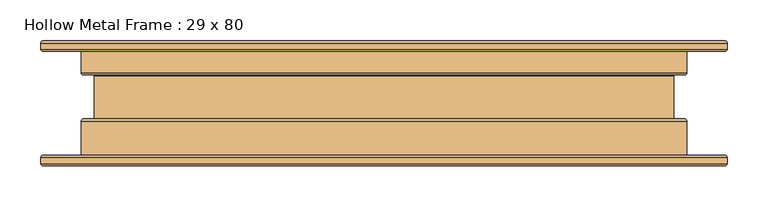
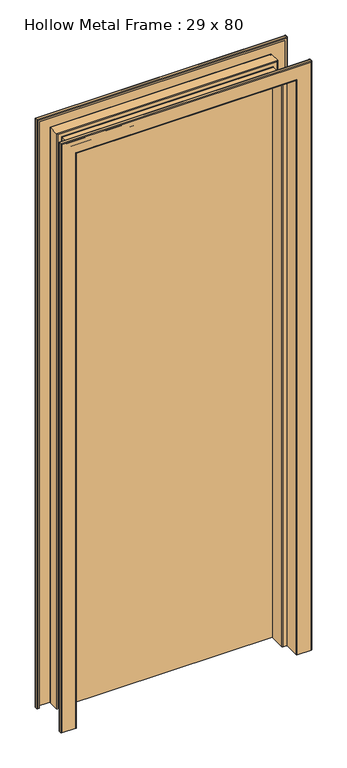
"""IFC4 building model written with IfcOpenShell, lengths in millimetres: door geometry, Hollow Metal Frame : 29 x 80."""

from ifc_helpers import new_model, si_unit, frame, origin, origin_with_axes, place, context, project, spatial, polyline, circle_curve, ellipse_curve, outline, extrude, source, transform, mapped, element, save
from ifc_brep_helpers import plane_surface, cylinder_surface, revolved_surface, advanced_brep


def hollow_metal_frame_29_x_80_a7873af5(model_context):
    return source(origin(), model_context, "Body", "SolidModel", [
        advanced_brep(
        [(-416.52825, -63.5635, 0.0), (-411.1625, -63.5635, 0.0), (-411.1625, -65.11925, 0.0), (-416.52825, -65.11925, 0.0), (-417.54425, -66.13525, 0.0), (-417.54425, -73.66, 0.0), (-416.52825, -74.676, 0.0), (-370.87175, -74.676, 0.0), (-369.85575, -73.66, 0.0), (-369.85575, -21.68525, 0.0), (-367.284, -19.1135, 0.0), (-354.99675, -19.1135, 0.0), (-353.98075, -18.0975, 0.0), (-353.98075, 33.6931, 0.0), (-354.99675, 34.7091, 0.0), (-367.284, 34.7091, 0.0), (-369.85575, 37.28085, 0.0), (-369.85575, 73.5965, 0.0), (-370.87175, 74.6125, 0.0), (-416.52825, 74.6125, 0.0), (-417.54425, 73.5965, 0.0), (-417.54425, 66.07175, 0.0), (-416.52825, 65.05575, 0.0), (-411.1625, 65.05575, 0.0), (-411.1625, 63.5, 0.0), (-416.52825, 63.5, 0.0), (-419.1, 66.07175, 0.0), (-419.1, 73.5965, 0.0), (-416.52825, 76.16825, 0.0), (-370.87175, 76.16825, 0.0), (-368.3, 73.5965, 0.0), (-368.3, 37.28085, 0.0), (-367.284, 36.26485, 0.0), (-354.99675, 36.26485, 0.0), (-352.425, 33.6931, 0.0), (-352.425, -18.0975, 0.0), (-354.99675, -20.66925, 0.0), (-367.284, -20.66925, 0.0), (-368.3, -21.68525, 0.0), (-368.3, -73.66, 0.0), (-370.87175, -76.23175, 0.0), (-416.52825, -76.23175, 0.0), (-419.1, -73.66, 0.0), (-419.1, -66.13525, 0.0), (-419.1, -66.13525, 2082.8000001), (-416.52825, -63.5635, 2080.2282501), (-419.1, -73.66, 2082.8000001), (-416.52825, -76.23175, 2080.2282501), (-370.87175, -76.23175, 2034.5717501), (370.87175, -76.23175, 2034.5717501), (370.87175, -76.23175, 0.0), (416.52825, -76.23175, 0.0), (416.52825, -76.23175, 2080.2282501), (-368.3, -73.66, 2032.0000001), (-368.3, -21.68525, 2032.0000001), (-367.284, -20.66925, 2030.9840001), (-354.99675, -20.66925, 2018.6967501), (354.99675, -20.66925, 2018.6967501), (354.99675, -20.66925, 0.0), (367.284, -20.66925, 0.0), (367.284, -20.66925, 2030.9840001), (-352.425, -18.0975, 2016.1250001), (-352.425, 33.6931, 2016.1250001), (-354.99675, 36.26485, 2018.6967501), (-367.284, 36.26485, 2030.9840001), (367.284, 36.26485, 2030.9840001), (367.284, 36.26485, 0.0), (354.99675, 36.26485, 0.0), (354.99675, 36.26485, 2018.6967501), (-368.3, 37.28085, 2032.0000001), (-368.3, 73.5965, 2032.0000001), (-370.87175, 76.16825, 2034.5717501), (-416.52825, 76.16825, 2080.2282501), (416.52825, 76.16825, 2080.2282501), (416.52825, 76.16825, 0.0), (370.87175, 76.16825, 0.0), (370.87175, 76.16825, 2034.5717501), (-419.1, 73.5965, 2082.8000001), (-419.1, 66.07175, 2082.8000001), (-416.52825, 63.5, 2080.2282501), (-411.1625, 63.5, 2074.8625001), (411.1625, 63.5, 2074.8625001), (411.1625, 63.5, 0.0), (416.52825, 63.5, 0.0), (416.52825, 63.5, 2080.2282501), (-411.1625, 65.05575, 2074.8625001), (-416.52825, 65.05575, 2080.2282501), (416.52825, 65.05575, 2080.2282501), (416.52825, 65.05575, 0.0), (411.1625, 65.05575, 0.0), (411.1625, 65.05575, 2074.8625001), (-417.54425, 66.07175, 2081.2442501), (-417.54425, 73.5965, 2081.2442501), (-416.52825, 74.6125, 2080.2282501), (-370.87175, 74.6125, 2034.5717501), (370.87175, 74.6125, 2034.5717501), (370.87175, 74.6125, 0.0), (416.52825, 74.6125, 0.0), (416.52825, 74.6125, 2080.2282501), (-369.85575, 73.5965, 2033.5557501), (-369.85575, 37.28085, 2033.5557501), (-367.284, 34.7091, 2030.9840001), (-354.99675, 34.7091, 2018.6967501), (354.99675, 34.7091, 2018.6967501), (354.99675, 34.7091, 0.0), (367.284, 34.7091, 0.0), (367.284, 34.7091, 2030.9840001), (-353.98075, 33.6931, 2017.6807501), (-353.98075, -18.0975, 2017.6807501), (-354.99675, -19.1135, 2018.6967501), (-367.284, -19.1135, 2030.9840001), (367.284, -19.1135, 2030.9840001), (367.284, -19.1135, 0.0), (354.99675, -19.1135, 0.0), (354.99675, -19.1135, 2018.6967501), (-369.85575, -21.68525, 2033.5557501), (-369.85575, -73.66, 2033.5557501), (-370.87175, -74.676, 2034.5717501), (-416.52825, -74.676, 2080.2282501), (416.52825, -74.676, 2080.2282501), (416.52825, -74.676, 0.0), (370.87175, -74.676, 0.0), (370.87175, -74.676, 2034.5717501), (-417.54425, -73.66, 2081.2442501), (-417.54425, -66.13525, 2081.2442501), (-416.52825, -65.11925, 2080.2282501), (-411.1625, -65.11925, 2074.8625001), (411.1625, -65.11925, 2074.8625001), (411.1625, -65.11925, 0.0), (416.52825, -65.11925, 0.0), (416.52825, -65.11925, 2080.2282501), (-411.1625, -63.5635, 2074.8625001), (416.52825, -63.5635, 2080.2282501), (416.52825, -63.5635, 0.0), (411.1625, -63.5635, 0.0), (411.1625, -63.5635, 2074.8625001), (419.1, -66.13525, 2082.8000001), (419.1, -73.66, 2082.8000001), (368.3, -73.66, 2032.0000001), (368.3, -21.68525, 2032.0000001), (352.425, -18.0975, 2016.1250001), (352.425, 33.6931, 2016.1250001), (368.3, 37.28085, 2032.0000001), (368.3, 73.5965, 2032.0000001), (419.1, 73.5965, 2082.8000001), (419.1, 66.07175, 2082.8000001), (417.54425, 66.07175, 2081.2442501), (417.54425, 73.5965, 2081.2442501), (369.85575, 73.5965, 2033.5557501), (369.85575, 37.28085, 2033.5557501), (353.98075, 33.6931, 2017.6807501), (353.98075, -18.0975, 2017.6807501), (369.85575, -21.68525, 2033.5557501), (369.85575, -73.66, 2033.5557501), (417.54425, -73.66, 2081.2442501), (417.54425, -66.13525, 2081.2442501), (419.1, -66.13525, 0.0), (419.1, -73.66, 0.0), (368.3, -73.66, 0.0), (368.3, -21.68525, 0.0), (352.425, -18.0975, 0.0), (352.425, 33.6931, 0.0), (368.3, 37.28085, 0.0), (368.3, 73.5965, 0.0), (419.1, 73.5965, 0.0), (419.1, 66.07175, 0.0), (417.54425, 66.07175, 0.0), (417.54425, 73.5965, 0.0), (369.85575, 73.5965, 0.0), (369.85575, 37.28085, 0.0), (353.98075, 33.6931, 0.0), (353.98075, -18.0975, 0.0), (369.85575, -21.68525, 0.0), (369.85575, -73.66, 0.0), (417.54425, -73.66, 0.0), (417.54425, -66.13525, 0.0)],
        [
            (0, 1),
            (1, 2),
            (2, 3),
            (3, 4, circle_curve(frame((-416.52825, -66.13525, 0.0), z_axis=(0.0, 0.0, 1.0), x_axis=(0.0, 1.0, 0.0)), 1.016)),
            (4, 5),
            (5, 6, circle_curve(frame((-416.52825, -73.66, 0.0), z_axis=(0.0, 0.0, 1.0), x_axis=(0.0, 1.0, 0.0)), 1.016)),
            (6, 7),
            (7, 8, circle_curve(frame((-370.87175, -73.66, 0.0), z_axis=(0.0, 0.0, 1.0), x_axis=(0.0, 1.0, 0.0)), 1.016)),
            (8, 9),
            (9, 10, circle_curve(frame((-367.284, -21.68525, 0.0), z_axis=(0.0, 0.0, -1.0), x_axis=(0.0, 1.0, 0.0)), 2.57175)),
            (10, 11),
            (11, 12, circle_curve(frame((-354.99675, -18.0975, 0.0), z_axis=(0.0, 0.0, 1.0), x_axis=(0.0, 1.0, 0.0)), 1.016)),
            (12, 13),
            (13, 14, circle_curve(frame((-354.99675, 33.6931, 0.0), z_axis=(0.0, 0.0, 1.0), x_axis=(0.0, 1.0, 0.0)), 1.016)),
            (14, 15),
            (15, 16, circle_curve(frame((-367.284, 37.28085, 0.0), z_axis=(0.0, 0.0, -1.0), x_axis=(0.0, 1.0, 0.0)), 2.57175)),
            (16, 17),
            (17, 18, circle_curve(frame((-370.87175, 73.5965, 0.0), z_axis=(0.0, 0.0, 1.0), x_axis=(0.0, 1.0, 0.0)), 1.016)),
            (18, 19),
            (19, 20, circle_curve(frame((-416.52825, 73.5965, 0.0), z_axis=(0.0, 0.0, 1.0), x_axis=(0.0, 1.0, 0.0)), 1.016)),
            (20, 21),
            (21, 22, circle_curve(frame((-416.52825, 66.07175, 0.0), z_axis=(0.0, 0.0, 1.0), x_axis=(0.0, 1.0, 0.0)), 1.016)),
            (22, 23),
            (23, 24),
            (24, 25),
            (25, 26, circle_curve(frame((-416.52825, 66.07175, 0.0), z_axis=(0.0, 0.0, -1.0), x_axis=(0.0, 1.0, 0.0)), 2.57175)),
            (26, 27),
            (27, 28, circle_curve(frame((-416.52825, 73.5965, 0.0), z_axis=(0.0, 0.0, -1.0), x_axis=(0.0, 1.0, 0.0)), 2.57175)),
            (28, 29),
            (29, 30, circle_curve(frame((-370.87175, 73.5965, 0.0), z_axis=(0.0, 0.0, -1.0), x_axis=(0.0, 1.0, 0.0)), 2.57175)),
            (30, 31),
            (31, 32, circle_curve(frame((-367.284, 37.28085, 0.0), z_axis=(0.0, 0.0, 1.0), x_axis=(0.0, 1.0, 0.0)), 1.016)),
            (32, 33),
            (33, 34, circle_curve(frame((-354.99675, 33.6931, 0.0), z_axis=(0.0, 0.0, -1.0), x_axis=(0.0, 1.0, 0.0)), 2.57175)),
            (34, 35),
            (35, 36, circle_curve(frame((-354.99675, -18.0975, 0.0), z_axis=(0.0, 0.0, -1.0), x_axis=(0.0, 1.0, 0.0)), 2.57175)),
            (36, 37),
            (37, 38, circle_curve(frame((-367.284, -21.68525, 0.0), z_axis=(0.0, 0.0, 1.0), x_axis=(0.0, 1.0, 0.0)), 1.016)),
            (38, 39),
            (39, 40, circle_curve(frame((-370.87175, -73.66, 0.0), z_axis=(0.0, 0.0, -1.0), x_axis=(0.0, 1.0, 0.0)), 2.57175)),
            (40, 41),
            (41, 42, circle_curve(frame((-416.52825, -73.66, 0.0), z_axis=(0.0, 0.0, -1.0), x_axis=(0.0, 1.0, 0.0)), 2.57175)),
            (42, 43),
            (43, 0, circle_curve(frame((-416.52825, -66.13525, 0.0), z_axis=(0.0, 0.0, -1.0), x_axis=(0.0, 1.0, 0.0)), 2.57175)),
            (43, 44),
            (44, 45, ellipse_curve(frame((-416.52825, -66.13525, 2080.2282501), z_axis=(-0.7071067811865475, 0.0, -0.7071067811865475), x_axis=(0.7071067811865474, 0.0, -0.7071067811865476)), 3.6370037, 2.57175)),
            (45, 0),
            (42, 46),
            (46, 44),
            (41, 47),
            (47, 46, ellipse_curve(frame((-416.52825, -73.66, 2080.2282501), z_axis=(-0.7071067811865475, 0.0, -0.7071067811865475), x_axis=(0.7071067811865474, 0.0, -0.7071067811865476)), 3.6370037, 2.57175)),
            (40, 48),
            (48, 49),
            (49, 50),
            (50, 51),
            (51, 52),
            (52, 47),
            (39, 53),
            (53, 48, ellipse_curve(frame((-370.87175, -73.66, 2034.5717501), z_axis=(-0.7071067811865475, 0.0, -0.7071067811865475), x_axis=(0.7071067811865474, 0.0, -0.7071067811865476)), 3.6370037, 2.57175)),
            (38, 54),
            (54, 53),
            (37, 55),
            (55, 54, ellipse_curve(frame((-367.284, -21.68525, 2030.9840001), z_axis=(0.7071067811865475, 0.0, 0.7071067811865475), x_axis=(-0.7071067811865474, 0.0, 0.7071067811865476)), 1.436841, 1.016)),
            (36, 56),
            (56, 57),
            (57, 58),
            (58, 59),
            (59, 60),
            (60, 55),
            (35, 61),
            (61, 56, ellipse_curve(frame((-354.99675, -18.0975, 2018.6967501), z_axis=(-0.7071067811865475, 0.0, -0.7071067811865475), x_axis=(0.7071067811865474, 0.0, -0.7071067811865476)), 3.6370037, 2.57175)),
            (34, 62),
            (62, 61),
            (33, 63),
            (63, 62, ellipse_curve(frame((-354.99675, 33.6931, 2018.6967501), z_axis=(-0.7071067811865475, 0.0, -0.7071067811865475), x_axis=(0.7071067811865474, 0.0, -0.7071067811865476)), 3.6370037, 2.57175)),
            (32, 64),
            (64, 65),
            (65, 66),
            (66, 67),
            (67, 68),
            (68, 63),
            (31, 69),
            (69, 64, ellipse_curve(frame((-367.284, 37.28085, 2030.9840001), z_axis=(0.7071067811865475, 0.0, 0.7071067811865475), x_axis=(-0.7071067811865474, 0.0, 0.7071067811865476)), 1.436841, 1.016)),
            (30, 70),
            (70, 69),
            (29, 71),
            (71, 70, ellipse_curve(frame((-370.87175, 73.5965, 2034.5717501), z_axis=(-0.7071067811865475, 0.0, -0.7071067811865475), x_axis=(0.7071067811865474, 0.0, -0.7071067811865476)), 3.6370037, 2.57175)),
            (28, 72),
            (72, 73),
            (73, 74),
            (74, 75),
            (75, 76),
            (76, 71),
            (27, 77),
            (77, 72, ellipse_curve(frame((-416.52825, 73.5965, 2080.2282501), z_axis=(-0.7071067811865475, 0.0, -0.7071067811865475), x_axis=(0.7071067811865474, 0.0, -0.7071067811865476)), 3.6370037, 2.57175)),
            (26, 78),
            (78, 77),
            (25, 79),
            (79, 78, ellipse_curve(frame((-416.52825, 66.07175, 2080.2282501), z_axis=(-0.7071067811865475, 0.0, -0.7071067811865475), x_axis=(0.7071067811865474, 0.0, -0.7071067811865476)), 3.6370037, 2.57175)),
            (24, 80),
            (80, 81),
            (81, 82),
            (82, 83),
            (83, 84),
            (84, 79),
            (23, 85),
            (85, 80),
            (22, 86),
            (86, 87),
            (87, 88),
            (88, 89),
            (89, 90),
            (90, 85),
            (21, 91),
            (91, 86, ellipse_curve(frame((-416.52825, 66.07175, 2080.2282501), z_axis=(0.7071067811865475, 0.0, 0.7071067811865475), x_axis=(-0.7071067811865474, 0.0, 0.7071067811865476)), 1.436841, 1.016)),
            (20, 92),
            (92, 91),
            (19, 93),
            (93, 92, ellipse_curve(frame((-416.52825, 73.5965, 2080.2282501), z_axis=(0.7071067811865475, 0.0, 0.7071067811865475), x_axis=(-0.7071067811865474, 0.0, 0.7071067811865476)), 1.436841, 1.016)),
            (18, 94),
            (94, 95),
            (95, 96),
            (96, 97),
            (97, 98),
            (98, 93),
            (17, 99),
            (99, 94, ellipse_curve(frame((-370.87175, 73.5965, 2034.5717501), z_axis=(0.7071067811865475, 0.0, 0.7071067811865475), x_axis=(-0.7071067811865474, 0.0, 0.7071067811865476)), 1.436841, 1.016)),
            (16, 100),
            (100, 99),
            (15, 101),
            (101, 100, ellipse_curve(frame((-367.284, 37.28085, 2030.9840001), z_axis=(-0.7071067811865475, 0.0, -0.7071067811865475), x_axis=(0.7071067811865474, 0.0, -0.7071067811865476)), 3.6370037, 2.57175)),
            (14, 102),
            (102, 103),
            (103, 104),
            (104, 105),
            (105, 106),
            (106, 101),
            (13, 107),
            (107, 102, ellipse_curve(frame((-354.99675, 33.6931, 2018.6967501), z_axis=(0.7071067811865475, 0.0, 0.7071067811865475), x_axis=(-0.7071067811865474, 0.0, 0.7071067811865476)), 1.436841, 1.016)),
            (12, 108),
            (108, 107),
            (11, 109),
            (109, 108, ellipse_curve(frame((-354.99675, -18.0975, 2018.6967501), z_axis=(0.7071067811865475, 0.0, 0.7071067811865475), x_axis=(-0.7071067811865474, 0.0, 0.7071067811865476)), 1.436841, 1.016)),
            (10, 110),
            (110, 111),
            (111, 112),
            (112, 113),
            (113, 114),
            (114, 109),
            (9, 115),
            (115, 110, ellipse_curve(frame((-367.284, -21.68525, 2030.9840001), z_axis=(-0.7071067811865475, 0.0, -0.7071067811865475), x_axis=(0.7071067811865474, 0.0, -0.7071067811865476)), 3.6370037, 2.57175)),
            (8, 116),
            (116, 115),
            (7, 117),
            (117, 116, ellipse_curve(frame((-370.87175, -73.66, 2034.5717501), z_axis=(0.7071067811865475, 0.0, 0.7071067811865475), x_axis=(-0.7071067811865474, 0.0, 0.7071067811865476)), 1.436841, 1.016)),
            (6, 118),
            (118, 119),
            (119, 120),
            (120, 121),
            (121, 122),
            (122, 117),
            (5, 123),
            (123, 118, ellipse_curve(frame((-416.52825, -73.66, 2080.2282501), z_axis=(0.7071067811865475, 0.0, 0.7071067811865475), x_axis=(-0.7071067811865474, 0.0, 0.7071067811865476)), 1.436841, 1.016)),
            (4, 124),
            (124, 123),
            (3, 125),
            (125, 124, ellipse_curve(frame((-416.52825, -66.13525, 2080.2282501), z_axis=(0.7071067811865475, 0.0, 0.7071067811865475), x_axis=(-0.7071067811865474, 0.0, 0.7071067811865476)), 1.436841, 1.016)),
            (2, 126),
            (126, 127),
            (127, 128),
            (128, 129),
            (129, 130),
            (130, 125),
            (1, 131),
            (131, 126),
            (45, 132),
            (132, 133),
            (133, 134),
            (134, 135),
            (135, 131),
            (44, 136),
            (136, 132, ellipse_curve(frame((416.52825, -66.13525, 2080.2282501), z_axis=(-0.7071067811865475, 0.0, 0.7071067811865475), x_axis=(-0.7071067811865476, 0.0, -0.7071067811865474)), 3.6370037, 2.57175)),
            (46, 137),
            (137, 136),
            (52, 137, ellipse_curve(frame((416.52825, -73.66, 2080.2282501), z_axis=(-0.7071067811865475, 0.0, 0.7071067811865475), x_axis=(-0.7071067811865476, 0.0, -0.7071067811865474)), 3.6370037, 2.57175)),
            (53, 138),
            (138, 49, ellipse_curve(frame((370.87175, -73.66, 2034.5717501), z_axis=(-0.7071067811865475, 0.0, 0.7071067811865475), x_axis=(-0.7071067811865476, 0.0, -0.7071067811865474)), 3.6370037, 2.57175)),
            (54, 139),
            (139, 138),
            (60, 139, ellipse_curve(frame((367.284, -21.68525, 2030.9840001), z_axis=(0.7071067811865475, 0.0, -0.7071067811865475), x_axis=(0.7071067811865476, 0.0, 0.7071067811865474)), 1.436841, 1.016)),
            (61, 140),
            (140, 57, ellipse_curve(frame((354.99675, -18.0975, 2018.6967501), z_axis=(-0.7071067811865475, 0.0, 0.7071067811865475), x_axis=(-0.7071067811865476, 0.0, -0.7071067811865474)), 3.6370037, 2.57175)),
            (62, 141),
            (141, 140),
            (68, 141, ellipse_curve(frame((354.99675, 33.6931, 2018.6967501), z_axis=(-0.7071067811865475, 0.0, 0.7071067811865475), x_axis=(-0.7071067811865476, 0.0, -0.7071067811865474)), 3.6370037, 2.57175)),
            (69, 142),
            (142, 65, ellipse_curve(frame((367.284, 37.28085, 2030.9840001), z_axis=(0.7071067811865475, 0.0, -0.7071067811865475), x_axis=(0.7071067811865476, 0.0, 0.7071067811865474)), 1.436841, 1.016)),
            (70, 143),
            (143, 142),
            (76, 143, ellipse_curve(frame((370.87175, 73.5965, 2034.5717501), z_axis=(-0.7071067811865475, 0.0, 0.7071067811865475), x_axis=(-0.7071067811865476, 0.0, -0.7071067811865474)), 3.6370037, 2.57175)),
            (77, 144),
            (144, 73, ellipse_curve(frame((416.52825, 73.5965, 2080.2282501), z_axis=(-0.7071067811865475, 0.0, 0.7071067811865475), x_axis=(-0.7071067811865476, 0.0, -0.7071067811865474)), 3.6370037, 2.57175)),
            (78, 145),
            (145, 144),
            (84, 145, ellipse_curve(frame((416.52825, 66.07175, 2080.2282501), z_axis=(-0.7071067811865475, 0.0, 0.7071067811865475), x_axis=(-0.7071067811865476, 0.0, -0.7071067811865474)), 3.6370037, 2.57175)),
            (90, 81),
            (91, 146),
            (146, 87, ellipse_curve(frame((416.52825, 66.07175, 2080.2282501), z_axis=(0.7071067811865475, 0.0, -0.7071067811865475), x_axis=(0.7071067811865476, 0.0, 0.7071067811865474)), 1.436841, 1.016)),
            (92, 147),
            (147, 146),
            (98, 147, ellipse_curve(frame((416.52825, 73.5965, 2080.2282501), z_axis=(0.7071067811865475, 0.0, -0.7071067811865475), x_axis=(0.7071067811865476, 0.0, 0.7071067811865474)), 1.436841, 1.016)),
            (99, 148),
            (148, 95, ellipse_curve(frame((370.87175, 73.5965, 2034.5717501), z_axis=(0.7071067811865475, 0.0, -0.7071067811865475), x_axis=(0.7071067811865476, 0.0, 0.7071067811865474)), 1.436841, 1.016)),
            (100, 149),
            (149, 148),
            (106, 149, ellipse_curve(frame((367.284, 37.28085, 2030.9840001), z_axis=(-0.7071067811865475, 0.0, 0.7071067811865475), x_axis=(-0.7071067811865476, 0.0, -0.7071067811865474)), 3.6370037, 2.57175)),
            (107, 150),
            (150, 103, ellipse_curve(frame((354.99675, 33.6931, 2018.6967501), z_axis=(0.7071067811865475, 0.0, -0.7071067811865475), x_axis=(0.7071067811865476, 0.0, 0.7071067811865474)), 1.436841, 1.016)),
            (108, 151),
            (151, 150),
            (114, 151, ellipse_curve(frame((354.99675, -18.0975, 2018.6967501), z_axis=(0.7071067811865475, 0.0, -0.7071067811865475), x_axis=(0.7071067811865476, 0.0, 0.7071067811865474)), 1.436841, 1.016)),
            (115, 152),
            (152, 111, ellipse_curve(frame((367.284, -21.68525, 2030.9840001), z_axis=(-0.7071067811865475, 0.0, 0.7071067811865475), x_axis=(-0.7071067811865476, 0.0, -0.7071067811865474)), 3.6370037, 2.57175)),
            (116, 153),
            (153, 152),
            (122, 153, ellipse_curve(frame((370.87175, -73.66, 2034.5717501), z_axis=(0.7071067811865475, 0.0, -0.7071067811865475), x_axis=(0.7071067811865476, 0.0, 0.7071067811865474)), 1.436841, 1.016)),
            (123, 154),
            (154, 119, ellipse_curve(frame((416.52825, -73.66, 2080.2282501), z_axis=(0.7071067811865475, 0.0, -0.7071067811865475), x_axis=(0.7071067811865476, 0.0, 0.7071067811865474)), 1.436841, 1.016)),
            (124, 155),
            (155, 154),
            (130, 155, ellipse_curve(frame((416.52825, -66.13525, 2080.2282501), z_axis=(0.7071067811865475, 0.0, -0.7071067811865475), x_axis=(0.7071067811865476, 0.0, 0.7071067811865474)), 1.436841, 1.016)),
            (135, 127),
            (133, 156, circle_curve(frame((416.52825, -66.13525, 0.0), z_axis=(0.0, 0.0, -1.0), x_axis=(0.0, 1.0, 0.0)), 2.57175)),
            (156, 157),
            (157, 51, circle_curve(frame((416.52825, -73.66, 0.0), z_axis=(0.0, 0.0, -1.0), x_axis=(0.0, 1.0, 0.0)), 2.57175)),
            (50, 158, circle_curve(frame((370.87175, -73.66, 0.0), z_axis=(0.0, 0.0, -1.0), x_axis=(0.0, 1.0, 0.0)), 2.57175)),
            (158, 159),
            (159, 59, circle_curve(frame((367.284, -21.68525, 0.0), z_axis=(0.0, 0.0, 1.0), x_axis=(0.0, 1.0, 0.0)), 1.016)),
            (58, 160, circle_curve(frame((354.99675, -18.0975, 0.0), z_axis=(0.0, 0.0, -1.0), x_axis=(0.0, 1.0, 0.0)), 2.57175)),
            (160, 161),
            (161, 67, circle_curve(frame((354.99675, 33.6931, 0.0), z_axis=(0.0, 0.0, -1.0), x_axis=(0.0, 1.0, 0.0)), 2.57175)),
            (66, 162, circle_curve(frame((367.284, 37.28085, 0.0), z_axis=(0.0, 0.0, 1.0), x_axis=(0.0, 1.0, 0.0)), 1.016)),
            (162, 163),
            (163, 75, circle_curve(frame((370.87175, 73.5965, 0.0), z_axis=(0.0, 0.0, -1.0), x_axis=(0.0, 1.0, 0.0)), 2.57175)),
            (74, 164, circle_curve(frame((416.52825, 73.5965, 0.0), z_axis=(0.0, 0.0, -1.0), x_axis=(0.0, 1.0, 0.0)), 2.57175)),
            (164, 165),
            (165, 83, circle_curve(frame((416.52825, 66.07175, 0.0), z_axis=(0.0, 0.0, -1.0), x_axis=(0.0, 1.0, 0.0)), 2.57175)),
            (82, 89),
            (88, 166, circle_curve(frame((416.52825, 66.07175, 0.0), z_axis=(0.0, 0.0, 1.0), x_axis=(0.0, 1.0, 0.0)), 1.016)),
            (166, 167),
            (167, 97, circle_curve(frame((416.52825, 73.5965, 0.0), z_axis=(0.0, 0.0, 1.0), x_axis=(0.0, 1.0, 0.0)), 1.016)),
            (96, 168, circle_curve(frame((370.87175, 73.5965, 0.0), z_axis=(0.0, 0.0, 1.0), x_axis=(0.0, 1.0, 0.0)), 1.016)),
            (168, 169),
            (169, 105, circle_curve(frame((367.284, 37.28085, 0.0), z_axis=(0.0, 0.0, -1.0), x_axis=(0.0, 1.0, 0.0)), 2.57175)),
            (104, 170, circle_curve(frame((354.99675, 33.6931, 0.0), z_axis=(0.0, 0.0, 1.0), x_axis=(0.0, 1.0, 0.0)), 1.016)),
            (170, 171),
            (171, 113, circle_curve(frame((354.99675, -18.0975, 0.0), z_axis=(0.0, 0.0, 1.0), x_axis=(0.0, 1.0, 0.0)), 1.016)),
            (112, 172, circle_curve(frame((367.284, -21.68525, 0.0), z_axis=(0.0, 0.0, -1.0), x_axis=(0.0, 1.0, 0.0)), 2.57175)),
            (172, 173),
            (173, 121, circle_curve(frame((370.87175, -73.66, 0.0), z_axis=(0.0, 0.0, 1.0), x_axis=(0.0, 1.0, 0.0)), 1.016)),
            (120, 174, circle_curve(frame((416.52825, -73.66, 0.0), z_axis=(0.0, 0.0, 1.0), x_axis=(0.0, 1.0, 0.0)), 1.016)),
            (174, 175),
            (175, 129, circle_curve(frame((416.52825, -66.13525, 0.0), z_axis=(0.0, 0.0, 1.0), x_axis=(0.0, 1.0, 0.0)), 1.016)),
            (128, 134),
            (136, 156),
            (137, 157),
            (138, 158),
            (139, 159),
            (140, 160),
            (141, 161),
            (142, 162),
            (143, 163),
            (144, 164),
            (145, 165),
            (146, 166),
            (147, 167),
            (148, 168),
            (149, 169),
            (150, 170),
            (151, 171),
            (152, 172),
            (153, 173),
            (154, 174),
            (155, 175),
        ],
        [
            plane_surface(frame((-379.4125, 63.5, 0.0), z_axis=(0.0, 0.0, -1.0), x_axis=(1.0, 0.0, 0.0))),
            cylinder_surface(frame((-416.52825, -66.13525, 0.0), z_axis=(0.0, 0.0, -1.0), x_axis=(0.0, 1.0, 0.0)), 2.57175),
            plane_surface(frame((-419.1, -66.13525, 0.0), z_axis=(-1.0, 0.0, 0.0), x_axis=(0.0, 0.0, 1.0))),
            cylinder_surface(frame((-416.52825, -73.66, 0.0), z_axis=(0.0, 0.0, -1.0), x_axis=(0.0, 1.0, 0.0)), 2.57175),
            plane_surface(frame((-416.52825, -76.23175, 0.0), z_axis=(0.0, -1.0, 0.0), x_axis=(0.0, 0.0, 1.0))),
            cylinder_surface(frame((-370.87175, -73.66, 0.0), z_axis=(0.0, 0.0, -1.0), x_axis=(0.0, 1.0, 0.0)), 2.57175),
            plane_surface(frame((-368.3, -73.66, 0.0), z_axis=(1.0, 0.0, 0.0), x_axis=(0.0, 0.0, 1.0))),
            revolved_surface(polyline([(-367.284, -20.669249999999998, 2032.0000001145868), (-367.284, -20.669249999999998, 0.0)]), (-367.284, -21.68525, 0.0), (0.0, 0.0, 1.0)),
            plane_surface(frame((-367.284, -20.66925, 0.0), z_axis=(0.0, -1.0, 0.0), x_axis=(0.0, 0.0, 1.0))),
            cylinder_surface(frame((-354.99675, -18.0975, 0.0), z_axis=(0.0, 0.0, -1.0), x_axis=(0.0, 1.0, 0.0)), 2.57175),
            plane_surface(frame((-352.425, -18.0975, 0.0), z_axis=(1.0, 0.0, 0.0), x_axis=(0.0, 0.0, 1.0))),
            cylinder_surface(frame((-354.99675, 33.6931, 0.0), z_axis=(0.0, 0.0, -1.0), x_axis=(0.0, 1.0, 0.0)), 2.57175),
            plane_surface(frame((-354.99675, 36.26485, 0.0), z_axis=(0.0, 1.0, 0.0), x_axis=(0.0, 0.0, 1.0))),
            revolved_surface(polyline([(-367.284, 38.29685, 2032.0000001145868), (-367.284, 38.29685, 0.0)]), (-367.284, 37.28085, 0.0), (0.0, 0.0, 1.0)),
            plane_surface(frame((-368.3, 37.28085, 0.0), z_axis=(1.0, 0.0, 0.0), x_axis=(0.0, 0.0, 1.0))),
            cylinder_surface(frame((-370.87175, 73.5965, 0.0), z_axis=(0.0, 0.0, -1.0), x_axis=(0.0, 1.0, 0.0)), 2.57175),
            plane_surface(frame((-370.87175, 76.16825, 0.0), z_axis=(0.0, 1.0, 0.0), x_axis=(0.0, 0.0, 1.0))),
            cylinder_surface(frame((-416.52825, 73.5965, 0.0), z_axis=(0.0, 0.0, -1.0), x_axis=(0.0, 1.0, 0.0)), 2.57175),
            plane_surface(frame((-419.1, 73.5965, 0.0), z_axis=(-1.0, 0.0, 0.0), x_axis=(0.0, 0.0, 1.0))),
            cylinder_surface(frame((-416.52825, 66.07175, 0.0), z_axis=(0.0, 0.0, -1.0), x_axis=(0.0, 1.0, 0.0)), 2.57175),
            plane_surface(frame((-416.52825, 63.5, 0.0), z_axis=(0.0, -1.0, 0.0), x_axis=(0.0, 0.0, 1.0))),
            plane_surface(frame((-411.1625, 63.5, 0.0), z_axis=(1.0, 0.0, 0.0), x_axis=(0.0, 0.0, 1.0))),
            plane_surface(frame((-411.1625, 65.05575, 0.0), z_axis=(0.0, 1.0, 0.0), x_axis=(0.0, 0.0, 1.0))),
            revolved_surface(polyline([(-416.52825, 67.08775, 2081.244250114587), (-416.52825, 67.08775, 0.0)]), (-416.52825, 66.07175, 0.0), (0.0, 0.0, 1.0)),
            plane_surface(frame((-417.54425, 66.07175, 0.0), z_axis=(1.0, 0.0, 0.0), x_axis=(0.0, 0.0, 1.0))),
            revolved_surface(polyline([(-416.52825, 74.61250000000001, 2081.244250114587), (-416.52825, 74.61250000000001, 0.0)]), (-416.52825, 73.5965, 0.0), (0.0, 0.0, 1.0)),
            plane_surface(frame((-416.52825, 74.6125, 0.0), z_axis=(0.0, -1.0, 0.0), x_axis=(0.0, 0.0, 1.0))),
            revolved_surface(polyline([(-370.87175, 74.61250000000001, 2035.5877501145867), (-370.87175, 74.61250000000001, 0.0)]), (-370.87175, 73.5965, 0.0), (0.0, 0.0, 1.0)),
            plane_surface(frame((-369.85575, 73.5965, 0.0), z_axis=(-1.0, 0.0, 0.0), x_axis=(0.0, 0.0, 1.0))),
            cylinder_surface(frame((-367.284, 37.28085, 0.0), z_axis=(0.0, 0.0, -1.0), x_axis=(0.0, 1.0, 0.0)), 2.57175),
            plane_surface(frame((-367.284, 34.7091, 0.0), z_axis=(0.0, -1.0, 0.0), x_axis=(0.0, 0.0, 1.0))),
            revolved_surface(polyline([(-354.99675, 34.7091, 2019.7127501145867), (-354.99675, 34.7091, 0.0)]), (-354.99675, 33.6931, 0.0), (0.0, 0.0, 1.0)),
            plane_surface(frame((-353.98075, 33.6931, 0.0), z_axis=(-1.0, 0.0, 0.0), x_axis=(0.0, 0.0, 1.0))),
            revolved_surface(polyline([(-354.99675, -17.0815, 2019.7127501145867), (-354.99675, -17.0815, 0.0)]), (-354.99675, -18.0975, 0.0), (0.0, 0.0, 1.0)),
            plane_surface(frame((-354.99675, -19.1135, 0.0), z_axis=(0.0, 1.0, 0.0), x_axis=(0.0, 0.0, 1.0))),
            cylinder_surface(frame((-367.284, -21.68525, 0.0), z_axis=(0.0, 0.0, -1.0), x_axis=(0.0, 1.0, 0.0)), 2.57175),
            plane_surface(frame((-369.85575, -21.68525, 0.0), z_axis=(-1.0, 0.0, 0.0), x_axis=(0.0, 0.0, 1.0))),
            revolved_surface(polyline([(-370.87175, -72.64399999999999, 2035.5877501145867), (-370.87175, -72.64399999999999, 0.0)]), (-370.87175, -73.66, 0.0), (0.0, 0.0, 1.0)),
            plane_surface(frame((-370.87175, -74.676, 0.0), z_axis=(0.0, 1.0, 0.0), x_axis=(0.0, 0.0, 1.0))),
            revolved_surface(polyline([(-416.52825, -72.64399999999999, 2081.244250114587), (-416.52825, -72.64399999999999, 0.0)]), (-416.52825, -73.66, 0.0), (0.0, 0.0, 1.0)),
            plane_surface(frame((-417.54425, -73.66, 0.0), z_axis=(1.0, 0.0, 0.0), x_axis=(0.0, 0.0, 1.0))),
            revolved_surface(polyline([(-416.52825, -65.11925, 2081.244250114587), (-416.52825, -65.11925, 0.0)]), (-416.52825, -66.13525, 0.0), (0.0, 0.0, 1.0)),
            plane_surface(frame((-416.52825, -65.11925, 0.0), z_axis=(0.0, -1.0, 0.0), x_axis=(0.0, 0.0, 1.0))),
            plane_surface(frame((-411.1625, -65.11925, 0.0), z_axis=(1.0, 0.0, 0.0), x_axis=(0.0, 0.0, 1.0))),
            plane_surface(frame((-411.1625, -63.5635, 0.0), z_axis=(0.0, 1.0, 0.0), x_axis=(0.0, 0.0, 1.0))),
            cylinder_surface(frame((-379.4125, -66.13525, 2080.2282501), z_axis=(-1.0, 0.0, 0.0), x_axis=(0.0, 1.0, 0.0)), 2.57175),
            plane_surface(frame((-419.1, -66.13525, 2082.8000001), z_axis=(0.0, 0.0, 1.0), x_axis=(1.0, 0.0, 0.0))),
            cylinder_surface(frame((-379.4125, -73.66, 2080.2282501), z_axis=(-1.0, 0.0, 0.0), x_axis=(0.0, 1.0, 0.0)), 2.57175),
            cylinder_surface(frame((-379.4125, -73.66, 2034.5717501), z_axis=(-1.0, 0.0, 0.0), x_axis=(0.0, 1.0, 0.0)), 2.57175),
            plane_surface(frame((-368.3, -73.66, 2032.0000001), z_axis=(0.0, 0.0, -1.0), x_axis=(1.0, 0.0, 0.0))),
            revolved_surface(polyline([(368.3000000145869, -20.669249999999998, 2030.9840001), (-368.30000001458683, -20.669249999999998, 2030.9840001)]), (-379.4125, -21.68525, 2030.9840001), (1.0, 0.0, 0.0)),
            cylinder_surface(frame((-379.4125, -18.0975, 2018.6967501), z_axis=(-1.0, 0.0, 0.0), x_axis=(0.0, 1.0, 0.0)), 2.57175),
            plane_surface(frame((-352.425, -18.0975, 2016.1250001), z_axis=(0.0, 0.0, -1.0), x_axis=(1.0, 0.0, 0.0))),
            cylinder_surface(frame((-379.4125, 33.6931, 2018.6967501), z_axis=(-1.0, 0.0, 0.0), x_axis=(0.0, 1.0, 0.0)), 2.57175),
            revolved_surface(polyline([(368.3000000145869, 38.29685, 2030.9840001), (-368.30000001458683, 38.29685, 2030.9840001)]), (-379.4125, 37.28085, 2030.9840001), (1.0, 0.0, 0.0)),
            plane_surface(frame((-368.3, 37.28085, 2032.0000001), z_axis=(0.0, 0.0, -1.0), x_axis=(1.0, 0.0, 0.0))),
            cylinder_surface(frame((-379.4125, 73.5965, 2034.5717501), z_axis=(-1.0, 0.0, 0.0), x_axis=(0.0, 1.0, 0.0)), 2.57175),
            cylinder_surface(frame((-379.4125, 73.5965, 2080.2282501), z_axis=(-1.0, 0.0, 0.0), x_axis=(0.0, 1.0, 0.0)), 2.57175),
            plane_surface(frame((-419.1, 73.5965, 2082.8000001), z_axis=(0.0, 0.0, 1.0), x_axis=(1.0, 0.0, 0.0))),
            cylinder_surface(frame((-379.4125, 66.07175, 2080.2282501), z_axis=(-1.0, 0.0, 0.0), x_axis=(0.0, 1.0, 0.0)), 2.57175),
            plane_surface(frame((-411.1625, 63.5, 2074.8625001), z_axis=(0.0, 0.0, -1.0), x_axis=(1.0, 0.0, 0.0))),
            revolved_surface(polyline([(417.54425001458685, 67.08775, 2080.2282501), (-417.54425001458685, 67.08775, 2080.2282501)]), (-379.4125, 66.07175, 2080.2282501), (1.0, 0.0, 0.0)),
            plane_surface(frame((-417.54425, 66.07175, 2081.2442501), z_axis=(0.0, 0.0, -1.0), x_axis=(1.0, 0.0, 0.0))),
            revolved_surface(polyline([(417.54425001458685, 74.61250000000001, 2080.2282501), (-417.54425001458685, 74.61250000000001, 2080.2282501)]), (-379.4125, 73.5965, 2080.2282501), (1.0, 0.0, 0.0)),
            revolved_surface(polyline([(371.8877500145869, 74.61250000000001, 2034.5717501), (-371.88775001458686, 74.61250000000001, 2034.5717501)]), (-379.4125, 73.5965, 2034.5717501), (1.0, 0.0, 0.0)),
            plane_surface(frame((-369.85575, 73.5965, 2033.5557501), z_axis=(0.0, 0.0, 1.0), x_axis=(1.0, 0.0, 0.0))),
            cylinder_surface(frame((-379.4125, 37.28085, 2030.9840001), z_axis=(-1.0, 0.0, 0.0), x_axis=(0.0, 1.0, 0.0)), 2.57175),
            revolved_surface(polyline([(356.0127500145869, 34.7091, 2018.6967501), (-356.01275001458686, 34.7091, 2018.6967501)]), (-379.4125, 33.6931, 2018.6967501), (1.0, 0.0, 0.0)),
            plane_surface(frame((-353.98075, 33.6931, 2017.6807501), z_axis=(0.0, 0.0, 1.0), x_axis=(1.0, 0.0, 0.0))),
            revolved_surface(polyline([(356.0127500145869, -17.0815, 2018.6967501), (-356.01275001458686, -17.0815, 2018.6967501)]), (-379.4125, -18.0975, 2018.6967501), (1.0, 0.0, 0.0)),
            cylinder_surface(frame((-379.4125, -21.68525, 2030.9840001), z_axis=(-1.0, 0.0, 0.0), x_axis=(0.0, 1.0, 0.0)), 2.57175),
            plane_surface(frame((-369.85575, -21.68525, 2033.5557501), z_axis=(0.0, 0.0, 1.0), x_axis=(1.0, 0.0, 0.0))),
            revolved_surface(polyline([(371.8877500145869, -72.64399999999999, 2034.5717501), (-371.88775001458686, -72.64399999999999, 2034.5717501)]), (-379.4125, -73.66, 2034.5717501), (1.0, 0.0, 0.0)),
            revolved_surface(polyline([(417.54425001458685, -72.64399999999999, 2080.2282501), (-417.54425001458685, -72.64399999999999, 2080.2282501)]), (-379.4125, -73.66, 2080.2282501), (1.0, 0.0, 0.0)),
            plane_surface(frame((-417.54425, -73.66, 2081.2442501), z_axis=(0.0, 0.0, -1.0), x_axis=(1.0, 0.0, 0.0))),
            revolved_surface(polyline([(417.54425001458685, -65.11925, 2080.2282501), (-417.54425001458685, -65.11925, 2080.2282501)]), (-379.4125, -66.13525, 2080.2282501), (1.0, 0.0, 0.0)),
            plane_surface(frame((-411.1625, -65.11925, 2074.8625001), z_axis=(0.0, 0.0, -1.0), x_axis=(1.0, 0.0, 0.0))),
            plane_surface(frame((379.4125, 63.5, 0.0), z_axis=(0.0, 0.0, -1.0), x_axis=(-1.0, 0.0, 0.0))),
            cylinder_surface(frame((416.52825, -66.13525, 2043.1125001), z_axis=(0.0, 0.0, 1.0), x_axis=(0.0, 1.0, 0.0)), 2.57175),
            plane_surface(frame((419.1, -66.13525, 2082.8000001), z_axis=(1.0, 0.0, 0.0), x_axis=(0.0, 0.0, -1.0))),
            cylinder_surface(frame((416.52825, -73.66, 2043.1125001), z_axis=(0.0, 0.0, 1.0), x_axis=(0.0, 1.0, 0.0)), 2.57175),
            cylinder_surface(frame((370.87175, -73.66, 2043.1125001), z_axis=(0.0, 0.0, 1.0), x_axis=(0.0, 1.0, 0.0)), 2.57175),
            plane_surface(frame((368.3, -73.66, 2032.0000001), z_axis=(-1.0, 0.0, 0.0), x_axis=(0.0, 0.0, -1.0))),
            revolved_surface(polyline([(367.284, -20.669249999999998, 0.0), (367.284, -20.669249999999998, 2032.0000001145868)]), (367.284, -21.68525, 2043.1125001), (0.0, 0.0, -1.0)),
            cylinder_surface(frame((354.99675, -18.0975, 2043.1125001), z_axis=(0.0, 0.0, 1.0), x_axis=(0.0, 1.0, 0.0)), 2.57175),
            plane_surface(frame((352.425, -18.0975, 2016.1250001), z_axis=(-1.0, 0.0, 0.0), x_axis=(0.0, 0.0, -1.0))),
            cylinder_surface(frame((354.99675, 33.6931, 2043.1125001), z_axis=(0.0, 0.0, 1.0), x_axis=(0.0, 1.0, 0.0)), 2.57175),
            revolved_surface(polyline([(367.284, 38.29685, 0.0), (367.284, 38.29685, 2032.0000001145868)]), (367.284, 37.28085, 2043.1125001), (0.0, 0.0, -1.0)),
            plane_surface(frame((368.3, 37.28085, 2032.0000001), z_axis=(-1.0, 0.0, 0.0), x_axis=(0.0, 0.0, -1.0))),
            cylinder_surface(frame((370.87175, 73.5965, 2043.1125001), z_axis=(0.0, 0.0, 1.0), x_axis=(0.0, 1.0, 0.0)), 2.57175),
            cylinder_surface(frame((416.52825, 73.5965, 2043.1125001), z_axis=(0.0, 0.0, 1.0), x_axis=(0.0, 1.0, 0.0)), 2.57175),
            plane_surface(frame((419.1, 73.5965, 2082.8000001), z_axis=(1.0, 0.0, 0.0), x_axis=(0.0, 0.0, -1.0))),
            cylinder_surface(frame((416.52825, 66.07175, 2043.1125001), z_axis=(0.0, 0.0, 1.0), x_axis=(0.0, 1.0, 0.0)), 2.57175),
            plane_surface(frame((411.1625, 63.5, 2074.8625001), z_axis=(-1.0, 0.0, 0.0), x_axis=(0.0, 0.0, -1.0))),
            revolved_surface(polyline([(416.52825, 67.08775, 0.0), (416.52825, 67.08775, 2081.244250114587)]), (416.52825, 66.07175, 2043.1125001), (0.0, 0.0, -1.0)),
            plane_surface(frame((417.54425, 66.07175, 2081.2442501), z_axis=(-1.0, 0.0, 0.0), x_axis=(0.0, 0.0, -1.0))),
            revolved_surface(polyline([(416.52825, 74.61250000000001, 0.0), (416.52825, 74.61250000000001, 2081.244250114587)]), (416.52825, 73.5965, 2043.1125001), (0.0, 0.0, -1.0)),
            revolved_surface(polyline([(370.87175, 74.61250000000001, 0.0), (370.87175, 74.61250000000001, 2035.5877501145867)]), (370.87175, 73.5965, 2043.1125001), (0.0, 0.0, -1.0)),
            plane_surface(frame((369.85575, 73.5965, 2033.5557501), z_axis=(1.0, 0.0, 0.0), x_axis=(0.0, 0.0, -1.0))),
            cylinder_surface(frame((367.284, 37.28085, 2043.1125001), z_axis=(0.0, 0.0, 1.0), x_axis=(0.0, 1.0, 0.0)), 2.57175),
            revolved_surface(polyline([(354.99675, 34.7091, 0.0), (354.99675, 34.7091, 2019.7127501145867)]), (354.99675, 33.6931, 2043.1125001), (0.0, 0.0, -1.0)),
            plane_surface(frame((353.98075, 33.6931, 2017.6807501), z_axis=(1.0, 0.0, 0.0), x_axis=(0.0, 0.0, -1.0))),
            revolved_surface(polyline([(354.99675, -17.0815, 0.0), (354.99675, -17.0815, 2019.7127501145867)]), (354.99675, -18.0975, 2043.1125001), (0.0, 0.0, -1.0)),
            cylinder_surface(frame((367.284, -21.68525, 2043.1125001), z_axis=(0.0, 0.0, 1.0), x_axis=(0.0, 1.0, 0.0)), 2.57175),
            plane_surface(frame((369.85575, -21.68525, 2033.5557501), z_axis=(1.0, 0.0, 0.0), x_axis=(0.0, 0.0, -1.0))),
            revolved_surface(polyline([(370.87175, -72.64399999999999, 0.0), (370.87175, -72.64399999999999, 2035.5877501145867)]), (370.87175, -73.66, 2043.1125001), (0.0, 0.0, -1.0)),
            revolved_surface(polyline([(416.52825, -72.64399999999999, 0.0), (416.52825, -72.64399999999999, 2081.244250114587)]), (416.52825, -73.66, 2043.1125001), (0.0, 0.0, -1.0)),
            plane_surface(frame((417.54425, -73.66, 2081.2442501), z_axis=(-1.0, 0.0, 0.0), x_axis=(0.0, 0.0, -1.0))),
            revolved_surface(polyline([(416.52825, -65.11925, 0.0), (416.52825, -65.11925, 2081.244250114587)]), (416.52825, -66.13525, 2043.1125001), (0.0, 0.0, -1.0)),
            plane_surface(frame((411.1625, -65.11925, 2074.8625001), z_axis=(-1.0, 0.0, 0.0), x_axis=(0.0, 0.0, -1.0))),
        ],
        [
            (0, [[1, 2, 3, 4, 5, 6, 7, 8, 9, 10, 11, 12, 13, 14, 15, 16, 17, 18, 19, 20, 21, 22, 23, 24, 25, 26, 27, 28, 29, 30, 31, 32, 33, 34, 35, 36, 37, 38, 39, 40, 41, 42, 43, 44]]),
            (1, [[45, 46, 47, -44]]),
            (2, [[48, 49, -45, -43]]),
            (3, [[50, 51, -48, -42]]),
            (4, [[52, 53, 54, 55, 56, 57, -50, -41]]),
            (5, [[58, 59, -52, -40]]),
            (6, [[60, 61, -58, -39]]),
            (7, [[62, 63, -60, -38]]),
            (8, [[64, 65, 66, 67, 68, 69, -62, -37]]),
            (9, [[70, 71, -64, -36]]),
            (10, [[72, 73, -70, -35]]),
            (11, [[74, 75, -72, -34]]),
            (12, [[76, 77, 78, 79, 80, 81, -74, -33]]),
            (13, [[82, 83, -76, -32]]),
            (14, [[84, 85, -82, -31]]),
            (15, [[86, 87, -84, -30]]),
            (16, [[88, 89, 90, 91, 92, 93, -86, -29]]),
            (17, [[94, 95, -88, -28]]),
            (18, [[96, 97, -94, -27]]),
            (19, [[98, 99, -96, -26]]),
            (20, [[100, 101, 102, 103, 104, 105, -98, -25]]),
            (21, [[106, 107, -100, -24]]),
            (22, [[108, 109, 110, 111, 112, 113, -106, -23]]),
            (23, [[114, 115, -108, -22]]),
            (24, [[116, 117, -114, -21]]),
            (25, [[118, 119, -116, -20]]),
            (26, [[120, 121, 122, 123, 124, 125, -118, -19]]),
            (27, [[126, 127, -120, -18]]),
            (28, [[128, 129, -126, -17]]),
            (29, [[130, 131, -128, -16]]),
            (30, [[132, 133, 134, 135, 136, 137, -130, -15]]),
            (31, [[138, 139, -132, -14]]),
            (32, [[140, 141, -138, -13]]),
            (33, [[142, 143, -140, -12]]),
            (34, [[144, 145, 146, 147, 148, 149, -142, -11]]),
            (35, [[150, 151, -144, -10]]),
            (36, [[152, 153, -150, -9]]),
            (37, [[154, 155, -152, -8]]),
            (38, [[156, 157, 158, 159, 160, 161, -154, -7]]),
            (39, [[162, 163, -156, -6]]),
            (40, [[164, 165, -162, -5]]),
            (41, [[166, 167, -164, -4]]),
            (42, [[168, 169, 170, 171, 172, 173, -166, -3]]),
            (43, [[174, 175, -168, -2]]),
            (44, [[-47, 176, 177, 178, 179, 180, -174, -1]]),
            (45, [[181, 182, -176, -46]]),
            (46, [[183, 184, -181, -49]]),
            (47, [[-57, 185, -183, -51]]),
            (48, [[186, 187, -53, -59]]),
            (49, [[188, 189, -186, -61]]),
            (50, [[-69, 190, -188, -63]]),
            (51, [[191, 192, -65, -71]]),
            (52, [[193, 194, -191, -73]]),
            (53, [[-81, 195, -193, -75]]),
            (54, [[196, 197, -77, -83]]),
            (55, [[198, 199, -196, -85]]),
            (56, [[-93, 200, -198, -87]]),
            (57, [[201, 202, -89, -95]]),
            (58, [[203, 204, -201, -97]]),
            (59, [[-105, 205, -203, -99]]),
            (60, [[-113, 206, -101, -107]]),
            (61, [[207, 208, -109, -115]]),
            (62, [[209, 210, -207, -117]]),
            (63, [[-125, 211, -209, -119]]),
            (64, [[212, 213, -121, -127]]),
            (65, [[214, 215, -212, -129]]),
            (66, [[-137, 216, -214, -131]]),
            (67, [[217, 218, -133, -139]]),
            (68, [[219, 220, -217, -141]]),
            (69, [[-149, 221, -219, -143]]),
            (70, [[222, 223, -145, -151]]),
            (71, [[224, 225, -222, -153]]),
            (72, [[-161, 226, -224, -155]]),
            (73, [[227, 228, -157, -163]]),
            (74, [[229, 230, -227, -165]]),
            (75, [[-173, 231, -229, -167]]),
            (76, [[-180, 232, -169, -175]]),
            (77, [[233, 234, 235, -55, 236, 237, 238, -67, 239, 240, 241, -79, 242, 243, 244, -91, 245, 246, 247, -103, 248, -111, 249, 250, 251, -123, 252, 253, 254, -135, 255, 256, 257, -147, 258, 259, 260, -159, 261, 262, 263, -171, 264, -178]]),
            (78, [[265, -233, -177, -182]]),
            (79, [[266, -234, -265, -184]]),
            (80, [[-56, -235, -266, -185]]),
            (81, [[267, -236, -54, -187]]),
            (82, [[268, -237, -267, -189]]),
            (83, [[-68, -238, -268, -190]]),
            (84, [[269, -239, -66, -192]]),
            (85, [[270, -240, -269, -194]]),
            (86, [[-80, -241, -270, -195]]),
            (87, [[271, -242, -78, -197]]),
            (88, [[272, -243, -271, -199]]),
            (89, [[-92, -244, -272, -200]]),
            (90, [[273, -245, -90, -202]]),
            (91, [[274, -246, -273, -204]]),
            (92, [[-104, -247, -274, -205]]),
            (93, [[-112, -248, -102, -206]]),
            (94, [[275, -249, -110, -208]]),
            (95, [[276, -250, -275, -210]]),
            (96, [[-124, -251, -276, -211]]),
            (97, [[277, -252, -122, -213]]),
            (98, [[278, -253, -277, -215]]),
            (99, [[-136, -254, -278, -216]]),
            (100, [[279, -255, -134, -218]]),
            (101, [[280, -256, -279, -220]]),
            (102, [[-148, -257, -280, -221]]),
            (103, [[281, -258, -146, -223]]),
            (104, [[282, -259, -281, -225]]),
            (105, [[-160, -260, -282, -226]]),
            (106, [[283, -261, -158, -228]]),
            (107, [[284, -262, -283, -230]]),
            (108, [[-172, -263, -284, -231]]),
            (109, [[-179, -264, -170, -232]]),
        ],
    ),
        extrude(outline(polyline([(366.74425, 37.28085), (-366.74425, 37.28085), (-366.74425, 63.5), (366.74425, 63.5), (366.74425, 37.28085)])), origin_with_axes(), (0.0, 0.0, 1.0), 2032.0000001),
    ])


if __name__ == "__main__":
    model = new_model("IFC4")
    model_context = context("Model", 3, world=origin())
    ifc_project = project(units=[si_unit("LENGTHUNIT", "METRE", prefix="MILLI")], contexts=[model_context])
    site = spatial("IfcSite", under=ifc_project)
    building = spatial("IfcBuilding", under=site)
    placement = place(None, origin())
    hollow_metal_frame_29_x_80_shape = hollow_metal_frame_29_x_80_a7873af5(model_context)
    element("IfcDoor", 1, ObjectType="Hollow Metal Frame : 29 x 80", at=placement, inside=building, context=model_context, shape_type="MappedRepresentation", body=[
        mapped(hollow_metal_frame_29_x_80_shape, transform((0.0, 0.0, 0.0), x_axis=(1.0, 0.0, 0.0), y_axis=(0.0, 1.0, 0.0), z_axis=(0.0, 0.0, 1.0))),
    ])
    save(model, "model.ifc")

# Revit data of these elements
# Type "Hollow Metal Frame : 29 x 80"
#   Type Mark = "v"
#   Product Page URL = ""
#   Product Name = ""
#   Product Documentation Link = ""
#   Material = ""
#   DS_Hardware_Set_(SFT) = ""
#   DS_Frame_Type_(SFT) = ""
#   DS_Fire_Rating_(SFT) = ""
#   DS_Door_Type_(SFT) = ""
#   Analytic Construction = "<None>"
#   Frame Projection Ext. = 0' - 1"
#   Frame Projection Int. = 0' - 1"
#   Frame Width = 0' - 3"
#   Height = 6' - 8"
#   Width = 2' - 5"
#   Non-Kerfed = yes
#   Kerfed = no
#   Hollow Metal Casing = Metal-Dunbarton_Doors-White
#   Flush Door = Metal-Dunbarton_Doors-Aluminum
#   DS_Frame_Material_(SFT) = none
#   DS_Door_Material_(SFT) = none
#   URL = ""
#   Model = ""
#   Manufacturer = ""
#   Function = (empty or 0)
#   Wall Closure = (empty or 0)
#   Description = (empty or 0)
# Element 1 (IfcDoor, "Hollow Metal Frame : 29 x 80")
#   Materials on its faces: "Metal-Dunbarton_Doors-White", "Metal-Dunbarton_Doors-Aluminum"
# Materials
#   "Metal-Dunbarton_Doors-White": class "Miscellaneous", colour RGB 230 233 236, transparency 0
#   "Metal-Dunbarton_Doors-Aluminum": class "System", colour RGB 143 142 141, transparency 0
